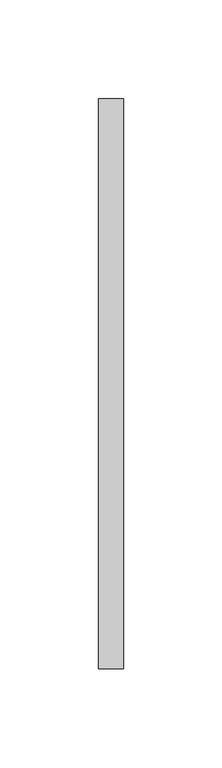
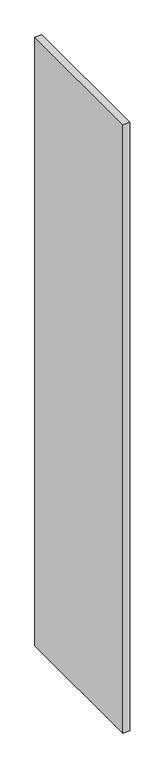
"""IFC4 building model written with IfcOpenShell, lengths in millimetres: proxy geometry, Inner panel:Inner panel:1:Inner panel:1 : Inner panel:Inner panel:300324:300043:Inner panel:1:Inner panel:1 : Inner panel:Inner panel:300324:300043 : Inner panel:Inner panel:1:Inner panel:1 : Inner panel:Inner panel:300324:300043:35 : Inner panel:Inner panel:1:Inner panel:1 : Inner panel:Inner panel:300324:300043:Inner panel:1:Inner panel:1 : Inner panel:Inner panel:300324:300043 : Inner panel:Inner panel:1:Inner panel:1 : Inner panel:Inner panel:300324:300043:300031."""

from ifc_helpers import new_model, si_unit, frame, origin, place, context, project, spatial, polyline, outline, extrude, source, transform, mapped, element, save


def generic_models_6cc5dbe0(model_context):
    return source(origin(), model_context, "Body", "SweptSolid", [
        extrude(outline(polyline([(579307.711724, -578724.4663841), (579320.4117239, -578724.4663841), (579320.4117239, -579013.3913841), (579307.711724, -579013.3913841), (579307.711724, -578724.4663841)])), frame((0.0, 0.0, 4946.65), z_axis=(0.0, 0.0, 1.0), x_axis=(1.0, 0.0, 0.0)), (0.0, 0.0, 1.0), 1219.2),
    ])


if __name__ == "__main__":
    model = new_model("IFC4")
    model_context = context("Model", 3, world=origin())
    ifc_project = project(units=[si_unit("LENGTHUNIT", "METRE", prefix="MILLI")], contexts=[model_context])
    site = spatial("IfcSite", under=ifc_project)
    building = spatial("IfcBuilding", under=site)
    placement = place(None, origin())
    generic_models_shape = generic_models_6cc5dbe0(model_context)
    element("IfcBuildingElementProxy", 1, Name="Inner panel:Inner panel:1:Inner panel:1 : Inner panel:Inner panel:300324:300043:Inner panel:1:Inner panel:1 : Inner panel:Inner panel:300324:300043 : Inner panel:Inner panel:1:Inner panel:1 : Inner panel:Inner panel:300324:300043:35 : Inner panel:Inner panel:1:Inner panel:1 : Inner panel:Inner panel:300324:300043:Inner panel:1:Inner panel:1 : Inner panel:Inner panel:300324:300043 : Inner panel:Inner panel:1:Inner panel:1 : Inner panel:Inner panel:300324:300043:300031", ObjectType="Inner panel:Inner panel:1:Inner panel:1 : Inner panel:Inner panel:300324:300043:Inner panel:1:Inner panel:1 : Inner panel:Inner panel:300324:300043 : Inner panel:Inner panel:1:Inner panel:1 : Inner panel:Inner panel:300324:300043:35 : Inner panel:Inner panel:1:Inner panel:1 : Inner panel:Inner panel:300324:300043:Inner panel:1:Inner panel:1 : Inner panel:Inner panel:300324:300043 : Inner panel:Inner panel:1:Inner panel:1 : Inner panel:Inner panel:300324:300043:300031", at=placement, inside=building, context=model_context, shape_type="MappedRepresentation", body=[
        mapped(generic_models_shape, transform((0.0, 0.0, 0.0), x_axis=(1.0, 0.0, 0.0), y_axis=(0.0, 1.0, 0.0), z_axis=(0.0, 0.0, 1.0))),
    ])
    save(model, "model.ifc")

# Revit data of these elements
# Type "Inner panel:Inner panel:1:Inner panel:1 : Inner panel:Inner panel:300324:300043:Inner panel:1:Inner panel:1 : Inner panel:Inner panel:300324:300043 : Inner panel:Inner panel:1:Inner panel:1 : Inner panel:Inner panel:300324:300043:35 : Inner panel:Inner panel:1:Inner panel:1 : Inner panel:Inner panel:300324:300043:Inner panel:1:Inner panel:1 : Inner panel:Inner panel:300324:300043 : Inner panel:Inner panel:1:Inner panel:1 : Inner panel:Inner panel:300324:300043:300031"
#   NameOverride = "Inner panel:Inner panel:1:Inner panel:1 : Inner panel:Inner panel:300324:300043:Inner panel:1:Inner panel:1 : Inner panel:Inner panel:300324:300043 : Inner panel:Inner panel:1:Inner panel:1 : Inner panel:Inner panel:300324:300043:300031"
#   ObjectTypeOverride = "Inner panel:1:Inner panel:1 : Inner panel:Inner panel:300324:300043 : Inner panel:Inner panel:1:Inner panel:1 : Inner panel:Inner panel:300324:300043"
#   Reference = "Inner panel"
#   Tag = "300031"
# Element 1 (IfcBuildingElementProxy, "Inner panel:Inner panel:1:Inner panel:1 : Inner panel:Inner panel:300324:300043:Inner panel:1:Inner panel:1 : Inner panel:Inner panel:300324:300043 : Inner panel:Inner panel:1:Inner panel:1 : Inner panel:Inner panel:300324:300043:35 : Inner panel:Inner panel:1:Inner panel:1 : Inner panel:Inner panel:300324:300043:Inner panel:1:Inner panel:1 : Inner panel:Inner panel:300324:300043 : Inner panel:Inner panel:1:Inner panel:1 : Inner panel:Inner panel:300324:300043:300031")
#   Materials on its faces: "1/2\" FIBERGLASS MAT GYPSUM PANELS"
# Materials
#   "1/2\" FIBERGLASS MAT GYPSUM PANELS": class "Generic", colour RGB 171 170 168, transparency 0, Description = "Gypsum Wall Board", Cost = 0
